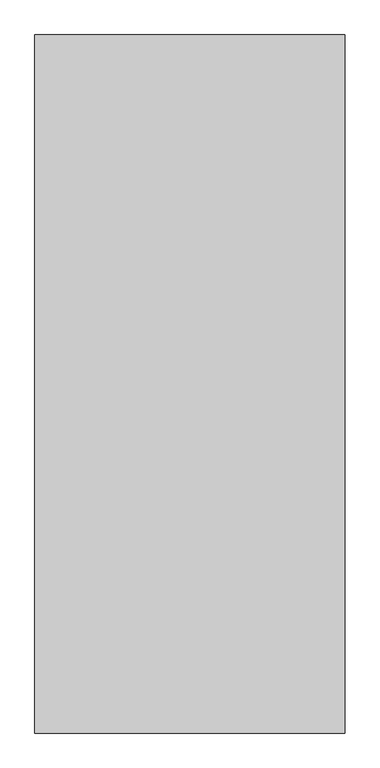
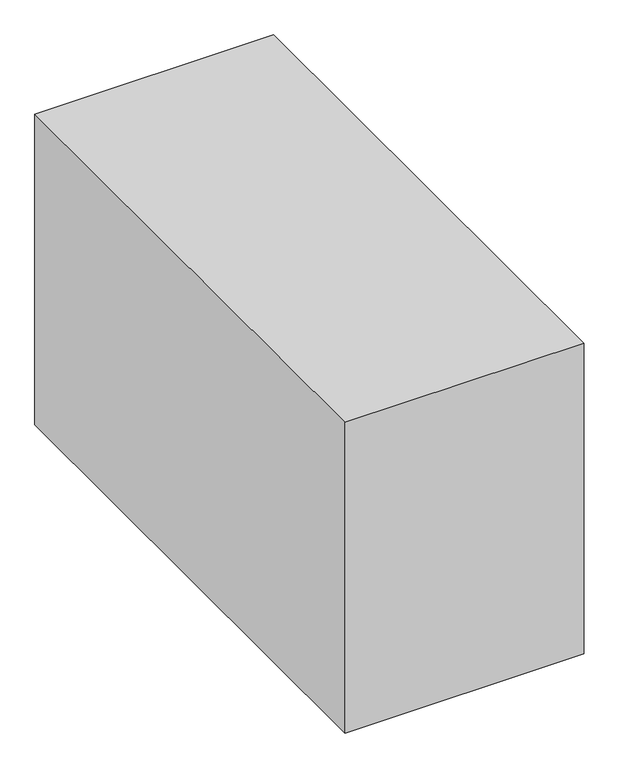
"""IFC4 building model written with IfcOpenShell, lengths in millimetres: proxy geometry, Space Planning Box_hec : Space Planning Box_hec."""

from ifc_helpers import new_model, si_unit, origin, origin_with_axes, place, context, project, spatial, polyline, outline, extrude, source, transform, mapped, element, save


def generic_models_8934d72c(model_context):
    return source(origin(), model_context, "Body", "SweptSolid", [
        extrude(outline(polyline([(2000.0, 4500.0), (2000.0, -4500.0), (-2000.0, -4500.0), (-2000.0, 4500.0), (2000.0, 4500.0)])), origin_with_axes(), (0.0, 0.0, 1.0), 5500.0),
    ])


if __name__ == "__main__":
    model = new_model("IFC4")
    model_context = context("Model", 3, world=origin())
    ifc_project = project(units=[si_unit("LENGTHUNIT", "METRE", prefix="MILLI")], contexts=[model_context])
    site = spatial("IfcSite", under=ifc_project)
    building = spatial("IfcBuilding", under=site)
    placement = place(None, origin())
    generic_models_shape = generic_models_8934d72c(model_context)
    element("IfcBuildingElementProxy", 1, Name="Space Planning Box_hec : Space Planning Box_hec", ObjectType="Space Planning Box_hec : Space Planning Box_hec", at=placement, inside=building, context=model_context, shape_type="MappedRepresentation", body=[
        mapped(generic_models_shape, transform((0.0, 0.0, 0.0), x_axis=(1.0, 0.0, 0.0), y_axis=(0.0, 1.0, 0.0), z_axis=(0.0, 0.0, 1.0))),
    ])
    save(model, "model.ifc")

# Revit data of these elements
# Type "Space Planning Box_hec : Space Planning Box_hec"
#   Type Comments = "..."
#   Room Name [instance default] = "?"
#   Interior Finish [instance default] = ""
#   Exterior Finish [instance default] = ""
#   Department [instance default] = ""
#   Assembly Code = "..."
#   ceiling height [instance default] = 0
#   Width [instance default] = 1524 mm
#   Program Area [instance default] = 0.00 m²
#   Length [instance default] = 1524 mm
#   Height [instance default] = 1524 mm
#   Area [instance default] = 2.32258 m²
#   Fill Color [instance default] = Cyan
#   Default Elevation = 0
# Element 1 (IfcBuildingElementProxy, "Space Planning Box_hec : Space Planning Box_hec")
#   Room Name = "Lobby"
#   Exterior Finish = "N/A..N/A,,EW2..N/A..N/A"
#   Department = "AR"
#   Width = 4000 mm
#   Program Area = 36.00 m²
#   Length = 9000 mm
#   Height = 5500 mm
#   Area = 36.00 m²
#   Materials on its faces: "Cyan"
# Materials
#   "Cyan": class "Generic", colour RGB 0 255 255, transparency 0.2, Cost = 0
